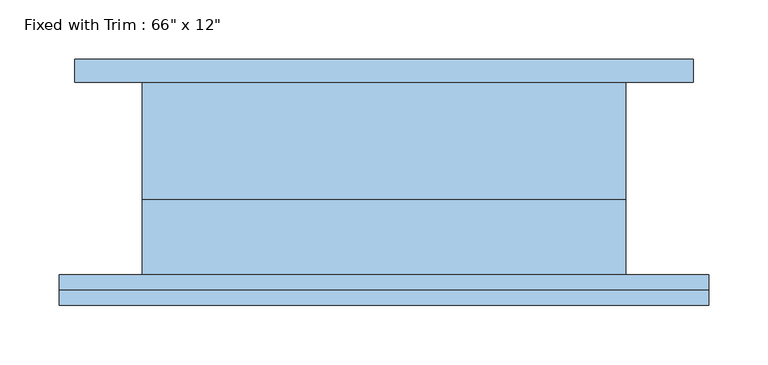
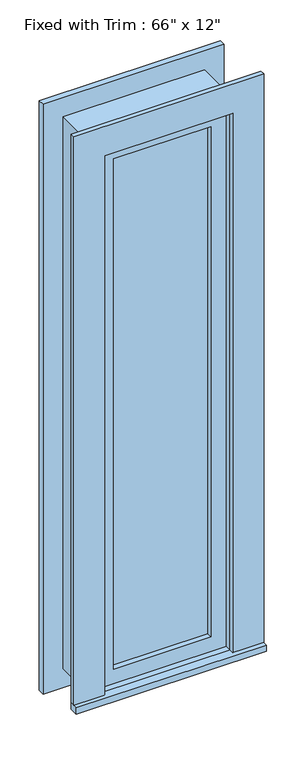
"""IFC4 building model written with IfcOpenShell, lengths in millimetres: window geometry."""

import ifcopenshell
import ifcopenshell.guid

model = None  # the IFC model being written
_history = None  # IfcOwnerHistory: only IFC2X3 demands one
_inside = {}  # id of a spatial element -> (the spatial element, [elements in it])
_under = {}  # id of a project, library or spatial element -> (it, [spatial elements below it])
_declared = {}  # id of a project -> (the project, [libraries it declares])
_typed = {}  # id of a type object -> (the type object, [elements of that type])
_made_of = {}  # id of a material, layer set ... -> (it, [elements and type objects made of it])


def new_model(schema):
    """Start an empty IFC model of exactly this schema.

    Asked for "IFC4X3", IfcOpenShell would pick the latest addendum, in which some entities
    have other attributes; the version numbers below select the first issue.
    IFC2X3 requires an IfcOwnerHistory on every rooted entity: one is made here for all.
    """
    global model, _history
    if schema == "IFC4X3":
        model = ifcopenshell.file(schema_version=(4, 3, 0, 0))
    else:
        model = ifcopenshell.file(schema=schema)
    _inside.clear()
    _under.clear()
    _declared.clear()
    _typed.clear()
    _made_of.clear()
    _history = None
    if model.schema == "IFC2X3":
        org = make("IfcOrganization", Name="unknown")
        user = make(
            "IfcPersonAndOrganization",
            ThePerson=make("IfcPerson", FamilyName="unknown"),
            TheOrganization=org,
        )
        app = make(
            "IfcApplication",
            ApplicationDeveloper=org,
            Version="unknown",
            ApplicationFullName="unknown",
            ApplicationIdentifier="unknown",
        )
        _history = make(
            "IfcOwnerHistory",
            OwningUser=user,
            OwningApplication=app,
            ChangeAction="ADDED",
            CreationDate=0,
        )
    return model


def make(cls, **values):
    """One entity of the class cls with the attributes given. An attribute that is None is left unset."""
    return model.create_entity(
        cls, **{name: value for name, value in values.items() if value is not None}
    )


def rooted(cls, **values):
    """An entity with a GlobalId (a new one), such as an element, a storey or a relation."""
    return make(cls, GlobalId=ifcopenshell.guid.new(), OwnerHistory=_history, **values)


def si_unit(unit_type, name, prefix=None):
    """IfcSIUnit, for example si_unit("LENGTHUNIT", "METRE", prefix="MILLI")."""
    return make("IfcSIUnit", UnitType=unit_type, Prefix=prefix, Name=name)


def assignment(units):
    """IfcUnitAssignment: the units of a project."""
    return None if units is None else make("IfcUnitAssignment", Units=units)


def point(xyz):
    """IfcCartesianPoint."""
    return None if xyz is None else make("IfcCartesianPoint", Coordinates=xyz)


def direction(xyz):
    """IfcDirection."""
    return None if xyz is None else make("IfcDirection", DirectionRatios=xyz)


def frame(location, z_axis=None, x_axis=None):
    """IfcAxis2Placement3D, a coordinate frame: its origin and axes. An axis left out is left unset."""
    return make(
        "IfcAxis2Placement3D",
        Location=point(location),
        Axis=direction(z_axis),
        RefDirection=direction(x_axis),
    )


def origin():
    """The frame at (0, 0, 0) with its axes left unset."""
    return frame((0.0, 0.0, 0.0))


def place(relative_to, where):
    """IfcLocalPlacement: puts the frame where relative to a parent placement (None: the world)."""
    return make(
        "IfcLocalPlacement", PlacementRelTo=relative_to, RelativePlacement=where
    )


def context(
    kind, dimensions, precision=None, world=None, true_north=None, identifier=None
):
    """IfcGeometricRepresentationContext, for example the 3D "Model" context."""
    return make(
        "IfcGeometricRepresentationContext",
        ContextIdentifier=identifier,
        ContextType=kind,
        CoordinateSpaceDimension=dimensions,
        Precision=precision,
        WorldCoordinateSystem=world,
        TrueNorth=true_north,
    )


def project(units=None, contexts=None):
    """IfcProject with its units and contexts."""
    return rooted(
        "IfcProject",
        Name="project",
        RepresentationContexts=contexts,
        UnitsInContext=assignment(units),
    )


def spatial(cls, under=None, at=None, **own):
    """A site, building, storey or space (cls), placed at a placement, below another one or the project."""
    s = rooted(cls, ObjectPlacement=at, **own)
    if under is not None:
        _under.setdefault(under.id(), (under, []))[1].append(s)
    return s


def polyline(points):
    """IfcPolyline through the points."""
    return make("IfcPolyline", Points=[point(p) for p in points])


def outline(outer, holes=None, kind="AREA"):
    """IfcArbitraryClosedProfileDef: a profile drawn as a closed curve; with holes, ...WithVoids."""
    if holes is None:
        return make("IfcArbitraryClosedProfileDef", ProfileType=kind, OuterCurve=outer)
    return make(
        "IfcArbitraryProfileDefWithVoids",
        ProfileType=kind,
        OuterCurve=outer,
        InnerCurves=holes,
    )


def extrude(swept, where, along, depth):
    """IfcExtrudedAreaSolid: the profile swept, set in the frame where, extruded along a direction by depth."""
    return make(
        "IfcExtrudedAreaSolid",
        SweptArea=swept,
        Position=where,
        ExtrudedDirection=direction(along),
        Depth=depth,
    )


def shape(context_of_items, identifier, shape_type, items):
    """IfcShapeRepresentation: the items that make up one representation, for example the "Body"."""
    return make(
        "IfcShapeRepresentation",
        ContextOfItems=context_of_items,
        RepresentationIdentifier=identifier,
        RepresentationType=shape_type,
        Items=items,
    )


def source(mapping_origin, context_of_items, identifier, shape_type, items):
    """IfcRepresentationMap: a shape defined once, which mapped items show again and again."""
    return make(
        "IfcRepresentationMap",
        MappingOrigin=mapping_origin,
        MappedRepresentation=shape(context_of_items, identifier, shape_type, items),
    )


def transform(
    local_origin,
    x_axis=None,
    y_axis=None,
    z_axis=None,
    scale=None,
    scale2=None,
    scale3=None,
    uniform=True,
):
    """IfcCartesianTransformationOperator3D, or its non-uniform kind. x_axis, y_axis, z_axis: its Axis1, 2, 3."""
    if uniform:
        return make(
            "IfcCartesianTransformationOperator3D",
            Axis1=direction(x_axis),
            Axis2=direction(y_axis),
            LocalOrigin=point(local_origin),
            Scale=scale,
            Axis3=direction(z_axis),
        )
    return make(
        "IfcCartesianTransformationOperator3DnonUniform",
        Axis1=direction(x_axis),
        Axis2=direction(y_axis),
        LocalOrigin=point(local_origin),
        Scale=scale,
        Axis3=direction(z_axis),
        Scale2=scale2,
        Scale3=scale3,
    )


def mapped(mapping_source, mapping_target):
    """IfcMappedItem: shows the shape of a source again, moved by a transform."""
    return make(
        "IfcMappedItem", MappingSource=mapping_source, MappingTarget=mapping_target
    )


def made_of(thing, what):
    """Note that an element or type object is made of a material, layer set ...; save() writes the relation."""
    if what is not None:
        _made_of.setdefault(what.id(), (what, []))[1].append(thing)
    return thing


def element(
    cls,
    number,
    at=None,
    inside=None,
    cuts=None,
    type_object=None,
    material=None,
    context=None,
    identifier="Body",
    shape_type=None,
    held_by="IfcProductDefinitionShape",
    body=None,
    shapes=None,
    **own,
):
    """One element of the class cls, such as IfcWall. Its Tag is "e" and its number.

    at: its placement. inside: the storey or other place that contains it. cuts: it is an
    opening in that element (IfcRelVoidsElement). A single representation is given by context,
    identifier, shape_type and body (its items); several are given by shapes. held_by: the class
    of the entity that holds the representations. save() writes the other relations.
    """
    e = rooted(cls, Tag="e%d" % number, ObjectPlacement=at, **own)
    if body is not None:
        shapes = [shape(context, identifier, shape_type, body)]
    if shapes is not None:
        e.Representation = make(held_by, Representations=shapes)
    if inside is not None:
        _inside.setdefault(inside.id(), (inside, []))[1].append(e)
    if cuts is not None:
        rooted(
            "IfcRelVoidsElement", RelatingBuildingElement=cuts, RelatedOpeningElement=e
        )
    if type_object is not None:
        _typed.setdefault(type_object.id(), (type_object, []))[1].append(e)
    return made_of(e, material)


def aggregate(whole, parts):
    """IfcRelAggregates: a whole, such as a stair, and the parts it consists of."""
    return rooted("IfcRelAggregates", RelatingObject=whole, RelatedObjects=parts)


def save(model, path):
    """Write the relations noted so far, then the file.

    IfcRelAggregates (storeys below a building ...), IfcRelContainedInSpatialStructure (elements
    in a storey), IfcRelDefinesByType, IfcRelAssociatesMaterial and IfcRelDeclares: one each for
    every whole, place, type object, material and project.
    """
    for whole, parts in _under.values():
        aggregate(whole, parts)
    for where, things in _inside.values():
        rooted(
            "IfcRelContainedInSpatialStructure",
            RelatedElements=things,
            RelatingStructure=where,
        )
    for kind, things in _typed.values():
        rooted("IfcRelDefinesByType", RelatedObjects=things, RelatingType=kind)
    for what, things in _made_of.values():
        rooted("IfcRelAssociatesMaterial", RelatedObjects=things, RelatingMaterial=what)
    for by, libraries in _declared.values():
        rooted("IfcRelDeclares", RelatingContext=by, RelatedDefinitions=libraries)
    model.write(path)


def window_2e97a10d(model_context):
    return source(origin(), model_context, "Body", "SweptSolid", [
        extrude(outline(polyline([(-311.15, -106.3625), (-311.15, -80.9625), (234.95, -80.9625), (234.95, -106.3625), (-311.15, -106.3625)])), frame((0.0, 0.0, 304.8), z_axis=(0.0, 0.0, 1.0), x_axis=(1.0, 0.0, 0.0)), (0.0, 0.0, 1.0), 19.05),
        extrude(outline(polyline([(1962.15, -222.25), (1962.15, 146.05), (323.85, 146.05), (323.85, 234.95), (2051.05, 234.95), (2051.05, -311.15), (323.85, -311.15), (323.85, -222.25), (1962.15, -222.25)])), frame((0.0, -93.6625, 0.0), z_axis=(0.0, 1.0, 0.0), x_axis=(0.0, 0.0, 1.0)), (0.0, 0.0, 1.0), 12.7),
        extrude(outline(polyline([(2038.35, 222.25), (2038.35, -298.45), (247.65, -298.45), (247.65, 222.25), (2038.35, 222.25)]), holes=[polyline([(1949.45, 133.35), (336.55, 133.35), (336.55, -209.55), (1949.45, -209.55), (1949.45, 133.35)])]), frame((0.0, 80.9625, 0.0), z_axis=(0.0, 1.0, 0.0), x_axis=(0.0, 0.0, 1.0)), (0.0, 0.0, 1.0), 19.05),
        extrude(outline(polyline([(101.6, -33.3375), (101.6, -46.0375), (-177.8, -46.0375), (-177.8, -33.3375), (101.6, -33.3375)])), frame((0.0, 0.0, 368.3), z_axis=(0.0, 0.0, 1.0), x_axis=(1.0, 0.0, 0.0)), (0.0, 0.0, 1.0), 1549.4),
        extrude(outline(polyline([(1962.15, -222.25), (323.85, -222.25), (323.85, 146.05), (1962.15, 146.05), (1962.15, -222.25)]), holes=[polyline([(1917.7, -177.8), (1917.7, 101.6), (368.3, 101.6), (368.3, -177.8), (1917.7, -177.8)])]), frame((0.0, -61.9125, 0.0), z_axis=(0.0, 1.0, 0.0), x_axis=(0.0, 0.0, 1.0)), (0.0, 0.0, 1.0), 44.45),
        extrude(outline(polyline([(1981.2, -241.3), (304.8, -241.3), (304.8, 165.1), (1981.2, 165.1), (1981.2, -241.3)]), holes=[polyline([(1949.45, -209.55), (1949.45, 133.35), (336.55, 133.35), (336.55, -209.55), (1949.45, -209.55)])]), frame((0.0, -17.4625, 0.0), z_axis=(0.0, 1.0, 0.0), x_axis=(0.0, 0.0, 1.0)), (0.0, 0.0, 1.0), 98.425),
        extrude(outline(polyline([(1981.2, 165.1), (1981.2, -241.3), (304.8, -241.3), (304.8, 165.1), (1981.2, 165.1)]), holes=[polyline([(1962.15, 146.05), (323.85, 146.05), (323.85, -222.25), (1962.15, -222.25), (1962.15, 146.05)])]), frame((0.0, -80.9625, 0.0), z_axis=(0.0, 1.0, 0.0), x_axis=(0.0, 0.0, 1.0)), (0.0, 0.0, 1.0), 63.5),
    ])


if __name__ == "__main__":
    model = new_model("IFC4")
    model_context = context("Model", 3, world=origin())
    ifc_project = project(units=[si_unit("LENGTHUNIT", "METRE", prefix="MILLI")], contexts=[model_context])
    site = spatial("IfcSite", under=ifc_project)
    building = spatial("IfcBuilding", under=site)
    placement = place(None, origin())
    window_shape = window_2e97a10d(model_context)
    element("IfcWindow", 1, ObjectType="Fixed with Trim : 66\" x 12\"", at=placement, inside=building, context=model_context, shape_type="MappedRepresentation", body=[
        mapped(window_shape, transform((0.0, 0.0, 0.0), x_axis=(1.0, 0.0, 0.0), y_axis=(0.0, 1.0, 0.0), z_axis=(0.0, 0.0, 1.0))),
    ])
    save(model, "model.ifc")

# Revit data of these elements
# Type "Fixed with Trim : 66\" x 12\""
#   Type Mark = "54"
#   COBie.Type.CreatedBy = "doug.wood@us.ibm.com"
#   COBie.Type.CreatedOn = "2016-04-14T02:07:26"
#   COBie.Type.Name = "Windows_Fixed with Trim_66\" x 12\"_54"
#   COBie.Type.Category = "23-30 20 17 11 : Fixed Windows"
#   COBie.Type.Description = "Fixed with Trim_66\" x 12\""
#   COBie.Type.Manufacturer = ""
#   COBie.Type.ModelNumber = ""
#   Construction Type Id = "GSP4R"
#   Assembly Code = "B2020100"
#   Analytic Construction = "1/8 in Pilkington single glazing"
#   COBie.Type.ReplacementCost = 0
#   Visual Light Transmittance = 0.9
#   Solar Heat Gain Coefficient = 0.78
#   Heat Transfer Coefficient (U) = 3.6886 W/(m²·K)
#   Height = 5' - 6"
#   Default Sill Height = 1' - 0"
#   Trim Projection - Ext. = 0' - 0 1/2"
#   Trim Projection - Int. = 0' - 0 3/4"
#   Trim Width - Exterior = 0' - 3 1/2"
#   Trim Width - Interior = 0' - 3 1/2"
#   Width = 1' - 4"
#   Window Inset = 0' - 0 3/4"
#   COBie.Type = no
#   Glass Pane Material = Glass
#   Sash Material = Sash - White
#   Trim Exterior Material = Trim - White
#   Trim Interior Material = Trim - White
#   Wall Closure = (empty or 0)
# Element 1 (IfcWindow, "Fixed with Trim : 66\" x 12\"")
#   Materials on its faces: "Sash - White", "Trim - White", "Glass"
# Materials
#   "Glass": class "Glass", colour RGB 0 128 192, transparency 0.75, Description = "Soda Lime Glass", Cost = 0
#   "Sash - White": class "Wood", colour RGB 255 255 255, transparency 0, Cost = 0
#   "Trim - White": class "Wood", colour RGB 255 255 255, transparency 0, Cost = 0
